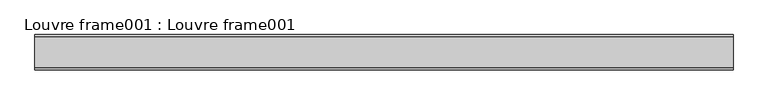
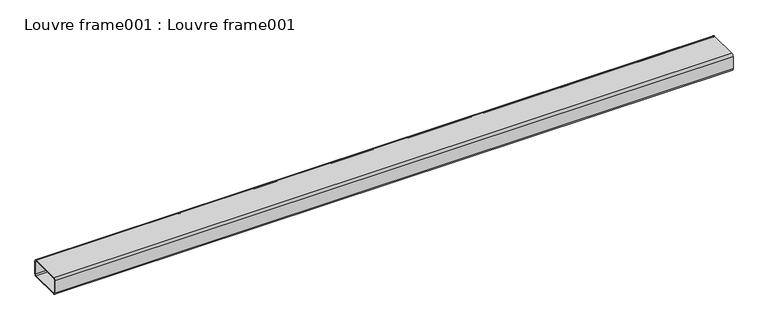
"""IFC4 building model written with IfcOpenShell, lengths in millimetres: proxy geometry, Louvre frame001 : Louvre frame001."""

from ifc_helpers import new_model, si_unit, point, frame, frame_2d, origin, place, context, project, spatial, polyline, circle_curve, trimmed, segment, composite_curve, outline, extrude, source, transform, mapped, element, save


def louvre_frame001_louvre_frame001_43cd0ce6(model_context):
    return source(origin(), model_context, "Body", "SweptSolid", [
        extrude(outline(composite_curve([segment(trimmed(circle_curve(frame_2d((9795.5719584, 37502.846)), 6.35), [point((9795.5719584, 37496.496))], [point((9789.2219584, 37502.846))], False, "CARTESIAN"), True, "CONTINUOUS"), segment(polyline([(9789.2219584, 37502.846), (9789.2219584, 37540.946)]), True, "CONTINUOUS"), segment(trimmed(circle_curve(frame_2d((9795.5719584, 37540.946)), 6.35), [point((9789.2219584, 37540.946))], [point((9795.5719584, 37547.296))], False, "CARTESIAN"), True, "CONTINUOUS"), segment(polyline([(9795.5719584, 37547.296), (9884.4719584, 37547.296)]), True, "CONTINUOUS"), segment(trimmed(circle_curve(frame_2d((9884.4719584, 37540.946)), 6.35), [point((9884.4719584, 37547.296))], [point((9890.8219584, 37540.946))], False, "CARTESIAN"), True, "CONTINUOUS"), segment(polyline([(9890.8219584, 37540.946), (9890.8219584, 37502.846)]), True, "CONTINUOUS"), segment(trimmed(circle_curve(frame_2d((9884.4719584, 37502.846)), 6.35), [point((9890.8219584, 37502.846))], [point((9884.4719584, 37496.496))], False, "CARTESIAN"), True, "CONTINUOUS"), segment(polyline([(9884.4719584, 37496.496), (9795.5719584, 37496.496)]), True, "CONTINUOUS")], self_intersect=False), holes=[composite_curve([segment(polyline([(9887.6519584, 37502.846), (9887.6519584, 37540.946)]), True, "CONTINUOUS"), segment(trimmed(circle_curve(frame_2d((9884.4719584, 37540.946)), 3.18), [point((9887.6519584, 37540.946))], [point((9884.4719584, 37544.126))], True, "CARTESIAN"), True, "CONTINUOUS"), segment(polyline([(9884.4719584, 37544.126), (9795.5719584, 37544.126)]), True, "CONTINUOUS"), segment(trimmed(circle_curve(frame_2d((9795.5719584, 37540.946)), 3.18), [point((9795.5719584, 37544.126))], [point((9792.3919584, 37540.946))], True, "CARTESIAN"), True, "CONTINUOUS"), segment(polyline([(9792.3919584, 37540.946), (9792.3919584, 37502.846)]), True, "CONTINUOUS"), segment(trimmed(circle_curve(frame_2d((9795.5719584, 37502.846)), 3.18), [point((9792.3919584, 37502.846))], [point((9795.5719584, 37499.666))], True, "CARTESIAN"), True, "CONTINUOUS"), segment(polyline([(9795.5719584, 37499.666), (9884.4719584, 37499.666)]), True, "CONTINUOUS"), segment(trimmed(circle_curve(frame_2d((9884.4719584, 37502.846)), 3.18), [point((9884.4719584, 37499.666))], [point((9887.6519584, 37502.846))], True, "CARTESIAN"), True, "CONTINUOUS")], self_intersect=False)]), frame((3694.2883192, 0.0, 0.0), z_axis=(1.0, 0.0, 0.0), x_axis=(0.0, 1.0, 0.0)), (0.0, 0.0, 1.0), 2000.0),
    ])


if __name__ == "__main__":
    model = new_model("IFC4")
    model_context = context("Model", 3, world=origin())
    ifc_project = project(units=[si_unit("LENGTHUNIT", "METRE", prefix="MILLI")], contexts=[model_context])
    site = spatial("IfcSite", under=ifc_project)
    building = spatial("IfcBuilding", under=site)
    placement = place(None, origin())
    louvre_frame001_louvre_frame001_shape = louvre_frame001_louvre_frame001_43cd0ce6(model_context)
    element("IfcBuildingElementProxy", 1, Name="Louvre frame001 : Louvre frame001", ObjectType="Louvre frame001 : Louvre frame001", at=placement, inside=building, context=model_context, shape_type="MappedRepresentation", body=[
        mapped(louvre_frame001_louvre_frame001_shape, transform((0.0, 0.0, 0.0), x_axis=(1.0, 0.0, 0.0), y_axis=(0.0, 1.0, 0.0), z_axis=(0.0, 0.0, 1.0))),
    ])
    save(model, "model.ifc")

# Revit data of these elements
# Type "Louvre frame001 : Louvre frame001"
#   NameOverride = "Louvre frame001"
# Element 1 (IfcBuildingElementProxy, "Louvre frame001 : Louvre frame001")
#   Materials on its faces: "ALUMINIUM LOUVER - TBD"
# Materials
#   "ALUMINIUM LOUVER - TBD": class "Unassigned", colour RGB 92 107 122, transparency 0, Cost = 0
